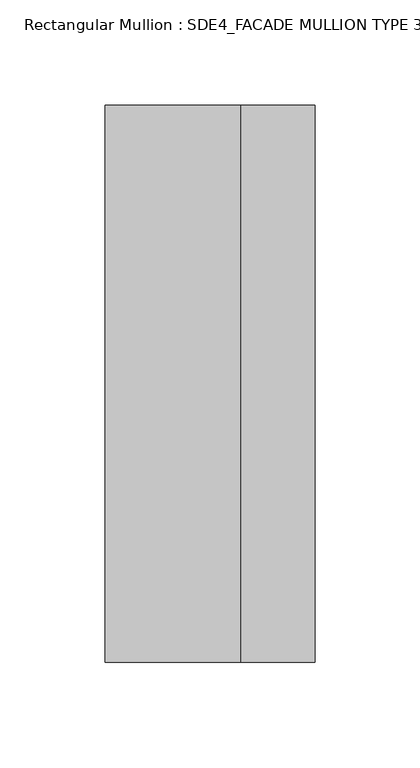
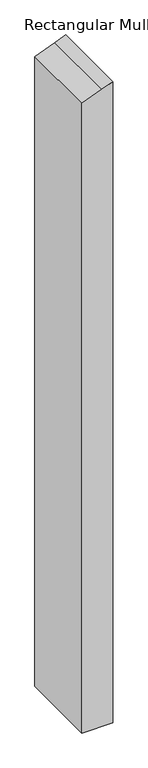
"""IFC4 building model written with IfcOpenShell, lengths in millimetres: member geometry, Rectangular Mullion : SDE4_FACADE MULLION TYPE 3."""

import ifcopenshell
import ifcopenshell.guid

model = None  # the IFC model being written
_history = None  # IfcOwnerHistory: only IFC2X3 demands one
_inside = {}  # id of a spatial element -> (the spatial element, [elements in it])
_under = {}  # id of a project, library or spatial element -> (it, [spatial elements below it])
_declared = {}  # id of a project -> (the project, [libraries it declares])
_typed = {}  # id of a type object -> (the type object, [elements of that type])
_made_of = {}  # id of a material, layer set ... -> (it, [elements and type objects made of it])


def new_model(schema):
    """Start an empty IFC model of exactly this schema.

    Asked for "IFC4X3", IfcOpenShell would pick the latest addendum, in which some entities
    have other attributes; the version numbers below select the first issue.
    IFC2X3 requires an IfcOwnerHistory on every rooted entity: one is made here for all.
    """
    global model, _history
    if schema == "IFC4X3":
        model = ifcopenshell.file(schema_version=(4, 3, 0, 0))
    else:
        model = ifcopenshell.file(schema=schema)
    _inside.clear()
    _under.clear()
    _declared.clear()
    _typed.clear()
    _made_of.clear()
    _history = None
    if model.schema == "IFC2X3":
        org = make("IfcOrganization", Name="unknown")
        user = make(
            "IfcPersonAndOrganization",
            ThePerson=make("IfcPerson", FamilyName="unknown"),
            TheOrganization=org,
        )
        app = make(
            "IfcApplication",
            ApplicationDeveloper=org,
            Version="unknown",
            ApplicationFullName="unknown",
            ApplicationIdentifier="unknown",
        )
        _history = make(
            "IfcOwnerHistory",
            OwningUser=user,
            OwningApplication=app,
            ChangeAction="ADDED",
            CreationDate=0,
        )
    return model


def make(cls, **values):
    """One entity of the class cls with the attributes given. An attribute that is None is left unset."""
    return model.create_entity(
        cls, **{name: value for name, value in values.items() if value is not None}
    )


def rooted(cls, **values):
    """An entity with a GlobalId (a new one), such as an element, a storey or a relation."""
    return make(cls, GlobalId=ifcopenshell.guid.new(), OwnerHistory=_history, **values)


def si_unit(unit_type, name, prefix=None):
    """IfcSIUnit, for example si_unit("LENGTHUNIT", "METRE", prefix="MILLI")."""
    return make("IfcSIUnit", UnitType=unit_type, Prefix=prefix, Name=name)


def assignment(units):
    """IfcUnitAssignment: the units of a project."""
    return None if units is None else make("IfcUnitAssignment", Units=units)


def point(xyz):
    """IfcCartesianPoint."""
    return None if xyz is None else make("IfcCartesianPoint", Coordinates=xyz)


def direction(xyz):
    """IfcDirection."""
    return None if xyz is None else make("IfcDirection", DirectionRatios=xyz)


def frame(location, z_axis=None, x_axis=None):
    """IfcAxis2Placement3D, a coordinate frame: its origin and axes. An axis left out is left unset."""
    return make(
        "IfcAxis2Placement3D",
        Location=point(location),
        Axis=direction(z_axis),
        RefDirection=direction(x_axis),
    )


def origin():
    """The frame at (0, 0, 0) with its axes left unset."""
    return frame((0.0, 0.0, 0.0))


def place(relative_to, where):
    """IfcLocalPlacement: puts the frame where relative to a parent placement (None: the world)."""
    return make(
        "IfcLocalPlacement", PlacementRelTo=relative_to, RelativePlacement=where
    )


def context(
    kind, dimensions, precision=None, world=None, true_north=None, identifier=None
):
    """IfcGeometricRepresentationContext, for example the 3D "Model" context."""
    return make(
        "IfcGeometricRepresentationContext",
        ContextIdentifier=identifier,
        ContextType=kind,
        CoordinateSpaceDimension=dimensions,
        Precision=precision,
        WorldCoordinateSystem=world,
        TrueNorth=true_north,
    )


def project(units=None, contexts=None):
    """IfcProject with its units and contexts."""
    return rooted(
        "IfcProject",
        Name="project",
        RepresentationContexts=contexts,
        UnitsInContext=assignment(units),
    )


def spatial(cls, under=None, at=None, **own):
    """A site, building, storey or space (cls), placed at a placement, below another one or the project."""
    s = rooted(cls, ObjectPlacement=at, **own)
    if under is not None:
        _under.setdefault(under.id(), (under, []))[1].append(s)
    return s


def polyline(points):
    """IfcPolyline through the points."""
    return make("IfcPolyline", Points=[point(p) for p in points])


def outline(outer, holes=None, kind="AREA"):
    """IfcArbitraryClosedProfileDef: a profile drawn as a closed curve; with holes, ...WithVoids."""
    if holes is None:
        return make("IfcArbitraryClosedProfileDef", ProfileType=kind, OuterCurve=outer)
    return make(
        "IfcArbitraryProfileDefWithVoids",
        ProfileType=kind,
        OuterCurve=outer,
        InnerCurves=holes,
    )


def extrude(swept, where, along, depth):
    """IfcExtrudedAreaSolid: the profile swept, set in the frame where, extruded along a direction by depth."""
    return make(
        "IfcExtrudedAreaSolid",
        SweptArea=swept,
        Position=where,
        ExtrudedDirection=direction(along),
        Depth=depth,
    )


def shape(context_of_items, identifier, shape_type, items):
    """IfcShapeRepresentation: the items that make up one representation, for example the "Body"."""
    return make(
        "IfcShapeRepresentation",
        ContextOfItems=context_of_items,
        RepresentationIdentifier=identifier,
        RepresentationType=shape_type,
        Items=items,
    )


def source(mapping_origin, context_of_items, identifier, shape_type, items):
    """IfcRepresentationMap: a shape defined once, which mapped items show again and again."""
    return make(
        "IfcRepresentationMap",
        MappingOrigin=mapping_origin,
        MappedRepresentation=shape(context_of_items, identifier, shape_type, items),
    )


def transform(
    local_origin,
    x_axis=None,
    y_axis=None,
    z_axis=None,
    scale=None,
    scale2=None,
    scale3=None,
    uniform=True,
):
    """IfcCartesianTransformationOperator3D, or its non-uniform kind. x_axis, y_axis, z_axis: its Axis1, 2, 3."""
    if uniform:
        return make(
            "IfcCartesianTransformationOperator3D",
            Axis1=direction(x_axis),
            Axis2=direction(y_axis),
            LocalOrigin=point(local_origin),
            Scale=scale,
            Axis3=direction(z_axis),
        )
    return make(
        "IfcCartesianTransformationOperator3DnonUniform",
        Axis1=direction(x_axis),
        Axis2=direction(y_axis),
        LocalOrigin=point(local_origin),
        Scale=scale,
        Axis3=direction(z_axis),
        Scale2=scale2,
        Scale3=scale3,
    )


def mapped(mapping_source, mapping_target):
    """IfcMappedItem: shows the shape of a source again, moved by a transform."""
    return make(
        "IfcMappedItem", MappingSource=mapping_source, MappingTarget=mapping_target
    )


def made_of(thing, what):
    """Note that an element or type object is made of a material, layer set ...; save() writes the relation."""
    if what is not None:
        _made_of.setdefault(what.id(), (what, []))[1].append(thing)
    return thing


def element(
    cls,
    number,
    at=None,
    inside=None,
    cuts=None,
    type_object=None,
    material=None,
    context=None,
    identifier="Body",
    shape_type=None,
    held_by="IfcProductDefinitionShape",
    body=None,
    shapes=None,
    **own,
):
    """One element of the class cls, such as IfcWall. Its Tag is "e" and its number.

    at: its placement. inside: the storey or other place that contains it. cuts: it is an
    opening in that element (IfcRelVoidsElement). A single representation is given by context,
    identifier, shape_type and body (its items); several are given by shapes. held_by: the class
    of the entity that holds the representations. save() writes the other relations.
    """
    e = rooted(cls, Tag="e%d" % number, ObjectPlacement=at, **own)
    if body is not None:
        shapes = [shape(context, identifier, shape_type, body)]
    if shapes is not None:
        e.Representation = make(held_by, Representations=shapes)
    if inside is not None:
        _inside.setdefault(inside.id(), (inside, []))[1].append(e)
    if cuts is not None:
        rooted(
            "IfcRelVoidsElement", RelatingBuildingElement=cuts, RelatedOpeningElement=e
        )
    if type_object is not None:
        _typed.setdefault(type_object.id(), (type_object, []))[1].append(e)
    return made_of(e, material)


def aggregate(whole, parts):
    """IfcRelAggregates: a whole, such as a stair, and the parts it consists of."""
    return rooted("IfcRelAggregates", RelatingObject=whole, RelatedObjects=parts)


def save(model, path):
    """Write the relations noted so far, then the file.

    IfcRelAggregates (storeys below a building ...), IfcRelContainedInSpatialStructure (elements
    in a storey), IfcRelDefinesByType, IfcRelAssociatesMaterial and IfcRelDeclares: one each for
    every whole, place, type object, material and project.
    """
    for whole, parts in _under.values():
        aggregate(whole, parts)
    for where, things in _inside.values():
        rooted(
            "IfcRelContainedInSpatialStructure",
            RelatedElements=things,
            RelatingStructure=where,
        )
    for kind, things in _typed.values():
        rooted("IfcRelDefinesByType", RelatedObjects=things, RelatingType=kind)
    for what, things in _made_of.values():
        rooted("IfcRelAssociatesMaterial", RelatedObjects=things, RelatingMaterial=what)
    for by, libraries in _declared.values():
        rooted("IfcRelDeclares", RelatingContext=by, RelatedDefinitions=libraries)
    model.write(path)


def rectangular_mullion_sde4_facade_mullion_type_3_fb4329d0(model_context):
    return source(origin(), model_context, "Body", "SweptSolid", [
        extrude(outline(polyline([(-23.0813185, 50.0), (-37.1390676, 14.8556271), (-63.0813185, -50.0), (-2227.974544, -50.0), (-2227.974544, 50.0), (-23.0813185, 50.0)])), frame((0.0, -132.5, 0.0), z_axis=(0.0, 1.0, 0.0), x_axis=(0.0, 0.0, 1.0)), (0.0, 0.0, 1.0), 265.0),
    ])


if __name__ == "__main__":
    model = new_model("IFC4")
    model_context = context("Model", 3, world=origin())
    ifc_project = project(units=[si_unit("LENGTHUNIT", "METRE", prefix="MILLI")], contexts=[model_context])
    site = spatial("IfcSite", under=ifc_project)
    building = spatial("IfcBuilding", under=site)
    placement = place(None, origin())
    rectangular_mullion_sde4_facade_mullion_type_3_shape = rectangular_mullion_sde4_facade_mullion_type_3_fb4329d0(model_context)
    element("IfcMember", 1, ObjectType="Rectangular Mullion : SDE4_FACADE MULLION TYPE 3", at=placement, inside=building, context=model_context, shape_type="MappedRepresentation", body=[
        mapped(rectangular_mullion_sde4_facade_mullion_type_3_shape, transform((0.0, 0.0, 0.0), x_axis=(1.0, 0.0, 0.0), y_axis=(0.0, 1.0, 0.0), z_axis=(0.0, 0.0, 1.0))),
    ])
    save(model, "model.ifc")

# Revit data of these elements
# Type "Rectangular Mullion : SDE4_FACADE MULLION TYPE 3"
#   built-in parameter 1007322 = 0.869423 (stored number, unit not read)
#   built-in parameter 1007321 = 0.164042 (stored number, unit not read)
#   built-in parameter 1007320 = 0.164042 (stored number, unit not read)
